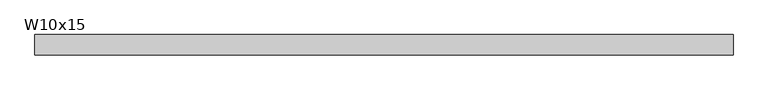
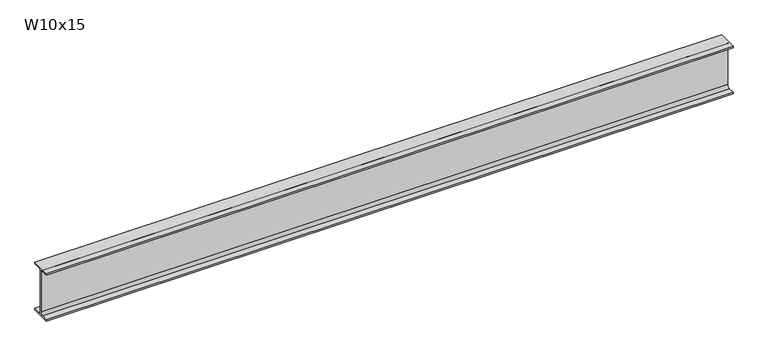
"""IFC4 building model written with IfcOpenShell, lengths in millimetres: beam geometry, RME W-Wide Flange : W10x15."""

from ifc_helpers import new_model, si_unit, point, frame, frame_2d, origin, place, context, project, spatial, polyline, circle_curve, trimmed, segment, composite_curve, outline, extrude, source, transform, mapped, element, save


def w10x15_42936043(model_context):
    return source(origin(), model_context, "Body", "SweptSolid", [
        extrude(outline(composite_curve([segment(polyline([(50.8, -120.142), (50.8, -127.0), (-50.8, -127.0), (-50.8, -120.142), (-16.7005, -120.142)]), True, "CONTINUOUS"), segment(trimmed(circle_curve(frame_2d((-16.7005, -106.3625)), 13.7795), [point((-16.7005, -120.142))], [point((-2.921, -106.3625))], True, "CARTESIAN"), True, "CONTINUOUS"), segment(polyline([(-2.921, -106.3625), (-2.921, 106.3625)]), True, "CONTINUOUS"), segment(trimmed(circle_curve(frame_2d((-16.7005, 106.3625)), 13.7795), [point((-2.921, 106.3625))], [point((-16.7005, 120.142))], True, "CARTESIAN"), True, "CONTINUOUS"), segment(polyline([(-16.7005, 120.142), (-50.8, 120.142), (-50.8, 127.0), (50.8, 127.0), (50.8, 120.142), (16.7005, 120.142)]), True, "CONTINUOUS"), segment(trimmed(circle_curve(frame_2d((16.7005, 106.3625)), 13.7795), [point((16.7005, 120.142))], [point((2.921, 106.3625))], True, "CARTESIAN"), True, "CONTINUOUS"), segment(polyline([(2.921, 106.3625), (2.921, -106.3625)]), True, "CONTINUOUS"), segment(trimmed(circle_curve(frame_2d((16.7005, -106.3625)), 13.7795), [point((2.921, -106.3625))], [point((16.7005, -120.142))], True, "CARTESIAN"), True, "CONTINUOUS"), segment(polyline([(16.7005, -120.142), (50.8, -120.142)]), True, "CONTINUOUS")], self_intersect=False)), frame((-1743.50793, 0.0, 0.0), z_axis=(1.0, 0.0, 0.0), x_axis=(0.0, 1.0, 0.0)), (0.0, 0.0, 1.0), 3487.01586),
    ])


if __name__ == "__main__":
    model = new_model("IFC4")
    model_context = context("Model", 3, world=origin())
    ifc_project = project(units=[si_unit("LENGTHUNIT", "METRE", prefix="MILLI")], contexts=[model_context])
    site = spatial("IfcSite", under=ifc_project)
    building = spatial("IfcBuilding", under=site)
    placement = place(None, origin())
    w10x15_shape = w10x15_42936043(model_context)
    element("IfcBeam", 1, ObjectType="RME W-Wide Flange : W10x15", at=placement, inside=building, context=model_context, shape_type="MappedRepresentation", body=[
        mapped(w10x15_shape, transform((0.0, 0.0, 0.0), x_axis=(1.0, 0.0, 0.0), y_axis=(0.0, 1.0, 0.0), z_axis=(0.0, 0.0, 1.0))),
    ])
    save(model, "model.ifc")

# Revit data of these elements
# Type "RME W-Wide Flange : W10x15"
#   WELD P [instance default] = ""
#   WELD LE [instance default] = ""
#   WELD D [instance default] = ""
#   TOP SECTION SIZE [instance default] = ""
#   TOP SECTION LENGTH [instance default] = ""
#   REMARKS [instance default] = ""
#   REINF TYPE [instance default] = ""
#   Nominal Size = "W24"
#   End Bearing Capacity [instance default] = ""
#   BOT SECTION SIZE [instance default] = ""
#   BOT SECTION LENGTH [instance default] = ""
#   Assembly Code = "B10"
#   W = 15
#   Start Extension Calculation [instance default] = 10' - 0"
#   Start Extension [instance default] = -0' - 0 1/2"
#   End Extension Calculation [instance default] = 10' - 0"
#   End Extension [instance default] = -0' - 0 1/2"
#   Length [instance default] = 5' - 0"
#   bf = 0' - 4"
#   d = 0' - 10"
#   k = 0' - 0 13/16"
#   k2 = 0' - 0.5425"
#   tf = 0' - 0.27"
#   tw = 0' - 0.23"
#   A = 0.030625 SF
#   Structural Material [instance default] = Metal - Steel - ASTM A992
# Element 1 (IfcBeam, "RME W-Wide Flange : W10x15")
#   Length = 11' - 5.28409"
#   Materials on its faces: "Metal - Steel - ASTM A992"
# Materials
#   "Metal - Steel - ASTM A992": class "Metal", colour RGB 255 128 0, transparency 0
